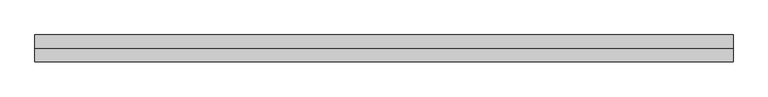
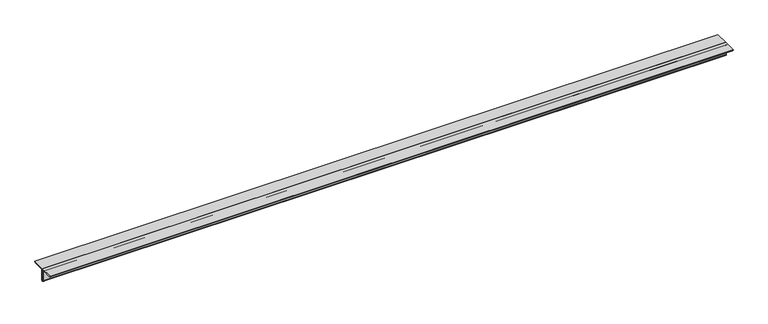
"""IFC4 building model written with IfcOpenShell, lengths in millimetres: member geometry, Steel Framing_2Ls_KS : H_SB_AR_S02_2Ls-100x100x10_VBR1."""

from ifc_helpers import new_model, si_unit, point, frame, frame_2d, origin, place, context, project, spatial, polyline, circle_curve, trimmed, segment, composite_curve, outline, extrude, source, transform, mapped, element, save


def member_26bf84cc(model_context):
    return source(origin(), model_context, "Body", "SweptSolid", [
        extrude(outline(composite_curve([segment(polyline([(0.0, 28.2), (100.0, 28.2)]), True, "CONTINUOUS"), segment(trimmed(circle_curve(frame_2d((90.0, 28.2)), 10.0), [point((100.0, 28.2))], [point((90.0, 18.2))], False, "CARTESIAN"), True, "CONTINUOUS"), segment(polyline([(90.0, 18.2), (20.0, 18.2)]), True, "CONTINUOUS"), segment(trimmed(circle_curve(frame_2d((20.0, 8.2)), 10.0), [point((20.0, 18.2))], [point((10.0, 8.2))], True, "CARTESIAN"), True, "CONTINUOUS"), segment(polyline([(10.0, 8.2), (10.0, -61.8)]), True, "CONTINUOUS"), segment(trimmed(circle_curve(frame_2d((0.0, -61.8)), 10.0), [point((10.0, -61.8))], [point((0.0, -71.8))], False, "CARTESIAN"), True, "CONTINUOUS"), segment(polyline([(0.0, -71.8), (0.0, 28.2)]), True, "CONTINUOUS")], self_intersect=False)), frame((-2590.3354834, 0.0, 0.0), z_axis=(1.0, 0.0, 0.0), x_axis=(0.0, 1.0, 0.0)), (0.0, 0.0, 1.0), 5195.0614478),
        extrude(outline(composite_curve([segment(polyline([(0.0, 28.2), (0.0, -71.8)]), True, "CONTINUOUS"), segment(trimmed(circle_curve(frame_2d((0.0, -61.8)), 10.0), [point((0.0, -71.8))], [point((-10.0, -61.8))], False, "CARTESIAN"), True, "CONTINUOUS"), segment(polyline([(-10.0, -61.8), (-10.0, 8.2)]), True, "CONTINUOUS"), segment(trimmed(circle_curve(frame_2d((-20.0, 8.2)), 10.0), [point((-10.0, 8.2))], [point((-20.0, 18.2))], True, "CARTESIAN"), True, "CONTINUOUS"), segment(polyline([(-20.0, 18.2), (-90.0, 18.2)]), True, "CONTINUOUS"), segment(trimmed(circle_curve(frame_2d((-90.0, 28.2)), 10.0), [point((-90.0, 18.2))], [point((-100.0, 28.2))], False, "CARTESIAN"), True, "CONTINUOUS"), segment(polyline([(-100.0, 28.2), (0.0, 28.2)]), True, "CONTINUOUS")], self_intersect=False)), frame((-2590.3354834, 0.0, 0.0), z_axis=(1.0, 0.0, 0.0), x_axis=(0.0, 1.0, 0.0)), (0.0, 0.0, 1.0), 5195.0614478),
    ])


if __name__ == "__main__":
    model = new_model("IFC4")
    model_context = context("Model", 3, world=origin())
    ifc_project = project(units=[si_unit("LENGTHUNIT", "METRE", prefix="MILLI")], contexts=[model_context])
    site = spatial("IfcSite", under=ifc_project)
    building = spatial("IfcBuilding", under=site)
    placement = place(None, origin())
    member_shape = member_26bf84cc(model_context)
    element("IfcMember", 1, ObjectType="Steel Framing_2Ls_KS : H_SB_AR_S02_2Ls-100x100x10_VBR1", at=placement, inside=building, context=model_context, shape_type="MappedRepresentation", body=[
        mapped(member_shape, transform((0.0, 0.0, 0.0), x_axis=(1.0, 0.0, 0.0), y_axis=(0.0, 1.0, 0.0), z_axis=(0.0, 0.0, 1.0))),
    ])
    save(model, "model.ifc")

# Revit data of these elements
# Type "Steel Framing_2Ls_KS : H_SB_AR_S02_2Ls-100x100x10_VBR1"
#   Type Comments = "MAIN"
#   Type Mark = "VBR1"
#   H_SectionID = "2Ls-100x100x10"
#   Assembly Code = "B10"
#   Legs = "LLBB"
#   H_Ratio for Additional Steel Plate = 0.2
#   W = 0
#   Perimeter = 0.80 m²/m
#   Nominal Weight = 29.80 kgf/m
#   Length [instance default] = 1524 mm
#   Space = 0 mm
#   b = 100 mm
#   d = 100 mm
#   t = 10 mm
#   y = 28.2 mm
#   A = 0.0038 m²
#   Structural Material [instance default] = Steel, 45-345
# Element 1 (IfcMember, "Steel Framing_2Ls_KS : H_SB_AR_S02_2Ls-100x100x10_VBR1")
#   Materials on its faces: "Steel, 45-345"
# Materials
#   "Steel, 45-345": class "Metal", colour RGB 189 187 185, transparency 0, Description = "Steel 345 MPa", Cost = 0
